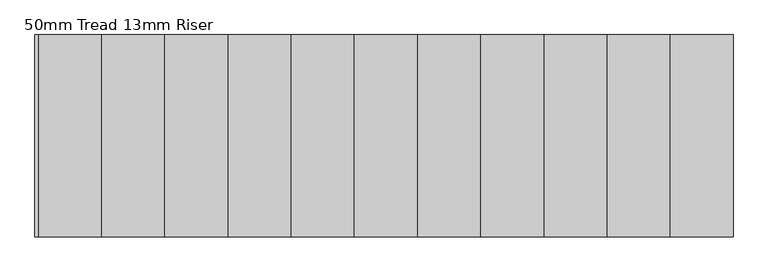
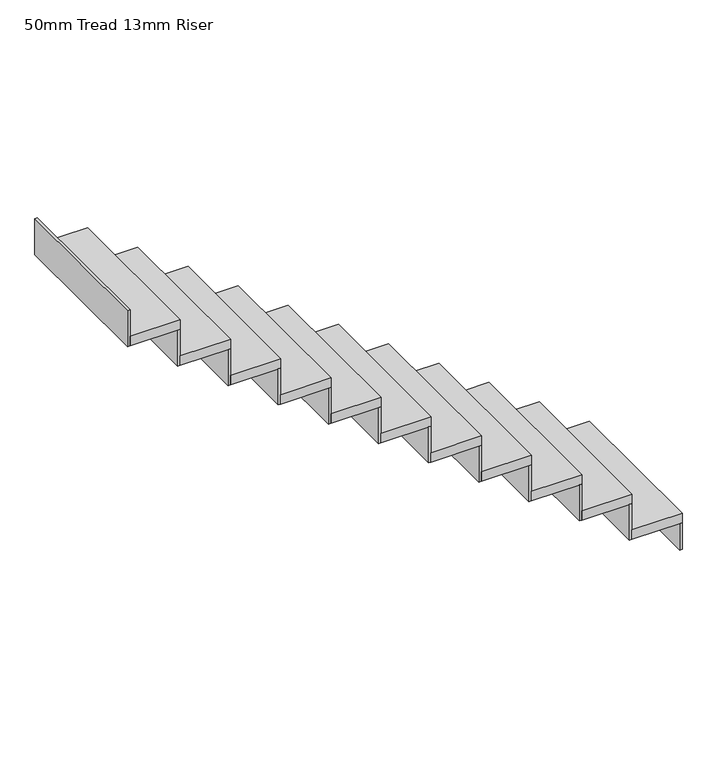
"""IFC4 building model written with IfcOpenShell, lengths in millimetres: stair flight geometry, 50mm Tread 13mm Riser."""

from ifc_helpers import new_model, si_unit, frame, origin, place, context, project, spatial, polyline, outline, extrude, source, transform, mapped, element, save


def stair_flight_50mm_tread_13mm_riser_2ca24aa0(model_context):
    return source(origin(), model_context, "Body", "SweptSolid", [
        extrude(outline(polyline([(-5062.9184352, 4472.0212329), (-5050.4184352, 4472.0212329), (-5050.4184352, 3672.0212329), (-5062.9184352, 3672.0212329), (-5062.9184352, 4472.0212329)])), frame((0.0, 0.0, 200.0), z_axis=(0.0, 0.0, 1.0), x_axis=(1.0, 0.0, 0.0)), (0.0, 0.0, 1.0), 139.3939394),
        extrude(outline(polyline([(-5300.4184352, 3672.0212329), (-5300.4184352, 4472.0212329), (-5050.4184352, 4472.0212329), (-5050.4184352, 3672.0212329), (-5300.4184352, 3672.0212329)])), frame((0.0, 0.0, 339.3939394), z_axis=(0.0, 0.0, 1.0), x_axis=(1.0, 0.0, 0.0)), (0.0, 0.0, 1.0), 50.0),
        extrude(outline(polyline([(-5312.9184352, 4472.0212329), (-5300.4184352, 4472.0212329), (-5300.4184352, 3672.0212329), (-5312.9184352, 3672.0212329), (-5312.9184352, 4472.0212329)])), frame((0.0, 0.0, 339.3939394), z_axis=(0.0, 0.0, 1.0), x_axis=(1.0, 0.0, 0.0)), (0.0, 0.0, 1.0), 189.3939394),
        extrude(outline(polyline([(-5550.4184352, 3672.0212329), (-5550.4184352, 4472.0212329), (-5300.4184352, 4472.0212329), (-5300.4184352, 3672.0212329), (-5550.4184352, 3672.0212329)])), frame((0.0, 0.0, 528.7878788), z_axis=(0.0, 0.0, 1.0), x_axis=(1.0, 0.0, 0.0)), (0.0, 0.0, 1.0), 50.0),
        extrude(outline(polyline([(-5562.9184352, 4472.0212329), (-5550.4184352, 4472.0212329), (-5550.4184352, 3672.0212329), (-5562.9184352, 3672.0212329), (-5562.9184352, 4472.0212329)])), frame((0.0, 0.0, 528.7878788), z_axis=(0.0, 0.0, 1.0), x_axis=(1.0, 0.0, 0.0)), (0.0, 0.0, 1.0), 189.3939394),
        extrude(outline(polyline([(-5800.4184352, 3672.0212329), (-5800.4184352, 4472.0212329), (-5550.4184352, 4472.0212329), (-5550.4184352, 3672.0212329), (-5800.4184352, 3672.0212329)])), frame((0.0, 0.0, 718.1818182), z_axis=(0.0, 0.0, 1.0), x_axis=(1.0, 0.0, 0.0)), (0.0, 0.0, 1.0), 50.0),
        extrude(outline(polyline([(-5812.9184352, 4472.0212329), (-5800.4184352, 4472.0212329), (-5800.4184352, 3672.0212329), (-5812.9184352, 3672.0212329), (-5812.9184352, 4472.0212329)])), frame((0.0, 0.0, 718.1818182), z_axis=(0.0, 0.0, 1.0), x_axis=(1.0, 0.0, 0.0)), (0.0, 0.0, 1.0), 189.3939394),
        extrude(outline(polyline([(-6050.4184352, 3672.0212329), (-6050.4184352, 4472.0212329), (-5800.4184352, 4472.0212329), (-5800.4184352, 3672.0212329), (-6050.4184352, 3672.0212329)])), frame((0.0, 0.0, 907.5757576), z_axis=(0.0, 0.0, 1.0), x_axis=(1.0, 0.0, 0.0)), (0.0, 0.0, 1.0), 50.0),
        extrude(outline(polyline([(-6062.9184352, 4472.0212329), (-6050.4184352, 4472.0212329), (-6050.4184352, 3672.0212329), (-6062.9184352, 3672.0212329), (-6062.9184352, 4472.0212329)])), frame((0.0, 0.0, 907.5757576), z_axis=(0.0, 0.0, 1.0), x_axis=(1.0, 0.0, 0.0)), (0.0, 0.0, 1.0), 189.3939394),
        extrude(outline(polyline([(-6300.4184352, 3672.0212329), (-6300.4184352, 4472.0212329), (-6050.4184352, 4472.0212329), (-6050.4184352, 3672.0212329), (-6300.4184352, 3672.0212329)])), frame((0.0, 0.0, 1096.969697), z_axis=(0.0, 0.0, 1.0), x_axis=(1.0, 0.0, 0.0)), (0.0, 0.0, 1.0), 50.0),
        extrude(outline(polyline([(-6312.9184352, 4472.0212329), (-6300.4184352, 4472.0212329), (-6300.4184352, 3672.0212329), (-6312.9184352, 3672.0212329), (-6312.9184352, 4472.0212329)])), frame((0.0, 0.0, 1096.969697), z_axis=(0.0, 0.0, 1.0), x_axis=(1.0, 0.0, 0.0)), (0.0, 0.0, 1.0), 189.3939394),
        extrude(outline(polyline([(-6550.4184352, 3672.0212329), (-6550.4184352, 4472.0212329), (-6300.4184352, 4472.0212329), (-6300.4184352, 3672.0212329), (-6550.4184352, 3672.0212329)])), frame((0.0, 0.0, 1286.3636364), z_axis=(0.0, 0.0, 1.0), x_axis=(1.0, 0.0, 0.0)), (0.0, 0.0, 1.0), 50.0),
        extrude(outline(polyline([(-6562.9184352, 4472.0212329), (-6550.4184352, 4472.0212329), (-6550.4184352, 3672.0212329), (-6562.9184352, 3672.0212329), (-6562.9184352, 4472.0212329)])), frame((0.0, 0.0, 1286.3636364), z_axis=(0.0, 0.0, 1.0), x_axis=(1.0, 0.0, 0.0)), (0.0, 0.0, 1.0), 189.3939394),
        extrude(outline(polyline([(-6800.4184352, 3672.0212329), (-6800.4184352, 4472.0212329), (-6550.4184352, 4472.0212329), (-6550.4184352, 3672.0212329), (-6800.4184352, 3672.0212329)])), frame((0.0, 0.0, 1475.7575758), z_axis=(0.0, 0.0, 1.0), x_axis=(1.0, 0.0, 0.0)), (0.0, 0.0, 1.0), 50.0),
        extrude(outline(polyline([(-6812.9184352, 4472.0212329), (-6800.4184352, 4472.0212329), (-6800.4184352, 3672.0212329), (-6812.9184352, 3672.0212329), (-6812.9184352, 4472.0212329)])), frame((0.0, 0.0, 1475.7575758), z_axis=(0.0, 0.0, 1.0), x_axis=(1.0, 0.0, 0.0)), (0.0, 0.0, 1.0), 189.3939394),
        extrude(outline(polyline([(-7050.4184352, 3672.0212329), (-7050.4184352, 4472.0212329), (-6800.4184352, 4472.0212329), (-6800.4184352, 3672.0212329), (-7050.4184352, 3672.0212329)])), frame((0.0, 0.0, 1665.1515152), z_axis=(0.0, 0.0, 1.0), x_axis=(1.0, 0.0, 0.0)), (0.0, 0.0, 1.0), 50.0),
        extrude(outline(polyline([(-7062.9184352, 4472.0212329), (-7050.4184352, 4472.0212329), (-7050.4184352, 3672.0212329), (-7062.9184352, 3672.0212329), (-7062.9184352, 4472.0212329)])), frame((0.0, 0.0, 1665.1515152), z_axis=(0.0, 0.0, 1.0), x_axis=(1.0, 0.0, 0.0)), (0.0, 0.0, 1.0), 189.3939394),
        extrude(outline(polyline([(-7300.4184352, 3672.0212329), (-7300.4184352, 4472.0212329), (-7050.4184352, 4472.0212329), (-7050.4184352, 3672.0212329), (-7300.4184352, 3672.0212329)])), frame((0.0, 0.0, 1854.5454545), z_axis=(0.0, 0.0, 1.0), x_axis=(1.0, 0.0, 0.0)), (0.0, 0.0, 1.0), 50.0),
        extrude(outline(polyline([(-7312.9184352, 4472.0212329), (-7300.4184352, 4472.0212329), (-7300.4184352, 3672.0212329), (-7312.9184352, 3672.0212329), (-7312.9184352, 4472.0212329)])), frame((0.0, 0.0, 1854.5454545), z_axis=(0.0, 0.0, 1.0), x_axis=(1.0, 0.0, 0.0)), (0.0, 0.0, 1.0), 189.3939394),
        extrude(outline(polyline([(-7550.4184352, 3672.0212329), (-7550.4184352, 4472.0212329), (-7300.4184352, 4472.0212329), (-7300.4184352, 3672.0212329), (-7550.4184352, 3672.0212329)])), frame((0.0, 0.0, 2043.9393939), z_axis=(0.0, 0.0, 1.0), x_axis=(1.0, 0.0, 0.0)), (0.0, 0.0, 1.0), 50.0),
        extrude(outline(polyline([(-7562.9184352, 4472.0212329), (-7550.4184352, 4472.0212329), (-7550.4184352, 3672.0212329), (-7562.9184352, 3672.0212329), (-7562.9184352, 4472.0212329)])), frame((0.0, 0.0, 2043.9393939), z_axis=(0.0, 0.0, 1.0), x_axis=(1.0, 0.0, 0.0)), (0.0, 0.0, 1.0), 189.3939394),
        extrude(outline(polyline([(-7812.9184352, 4472.0212329), (-7800.4184352, 4472.0212329), (-7800.4184352, 3672.0212329), (-7812.9184352, 3672.0212329), (-7812.9184352, 4472.0212329)])), frame((0.0, 0.0, 2233.3333333), z_axis=(0.0, 0.0, 1.0), x_axis=(1.0, 0.0, 0.0)), (0.0, 0.0, 1.0), 189.3939394),
        extrude(outline(polyline([(-7800.4184352, 3672.0212329), (-7800.4184352, 4472.0212329), (-7550.4184352, 4472.0212329), (-7550.4184352, 3672.0212329), (-7800.4184352, 3672.0212329)])), frame((0.0, 0.0, 2233.3333333), z_axis=(0.0, 0.0, 1.0), x_axis=(1.0, 0.0, 0.0)), (0.0, 0.0, 1.0), 50.0),
    ])


if __name__ == "__main__":
    model = new_model("IFC4")
    model_context = context("Model", 3, world=origin())
    ifc_project = project(units=[si_unit("LENGTHUNIT", "METRE", prefix="MILLI")], contexts=[model_context])
    site = spatial("IfcSite", under=ifc_project)
    building = spatial("IfcBuilding", under=site)
    placement = place(None, origin())
    stair_flight_50mm_tread_13mm_riser_shape = stair_flight_50mm_tread_13mm_riser_2ca24aa0(model_context)
    element("IfcStairFlight", 1, ObjectType="50mm Tread 13mm Riser", at=placement, inside=building, context=model_context, shape_type="MappedRepresentation", body=[
        mapped(stair_flight_50mm_tread_13mm_riser_shape, transform((0.0, 0.0, 0.0), x_axis=(1.0, 0.0, 0.0), y_axis=(0.0, 1.0, 0.0), z_axis=(0.0, 0.0, 1.0))),
    ])
    save(model, "model.ifc")
